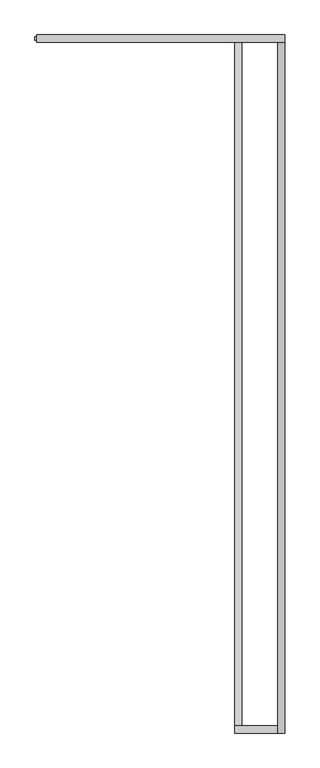
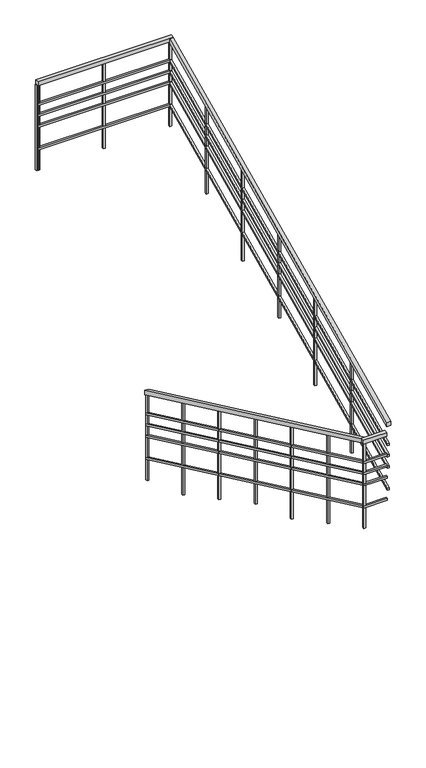
"""IFC4 building model written with IfcOpenShell, lengths in millimetres: railing geometry."""

from ifc_helpers import new_model, si_unit, frame, origin, place, context, project, spatial, polyline, outline, extrude, source, transform, mapped, element, save


def railing_ccc11bfa(model_context):
    return source(origin(), model_context, "Body", "SweptSolid", [
        extrude(outline(polyline([(4259.5597612, 1346.4361595), (4259.5597612, 1291.1764706), (-515.4402388, 3538.2352941), (-515.4402388, 3593.494983), (4259.5597612, 1346.4361595)])), frame((14225.0, 0.0, 0.0), z_axis=(1.0, 0.0, 0.0), x_axis=(0.0, 1.0, 0.0)), (0.0, 0.0, 1.0), 50.0),
        extrude(outline(polyline([(14225.0, -565.4402388), (14225.0, -515.4402388), (14525.0, -515.4402388), (14525.0, -565.4402388), (14225.0, -565.4402388)])), frame((0.0, 0.0, 3550.0), z_axis=(0.0, 0.0, 1.0), x_axis=(1.0, 0.0, 0.0)), (0.0, 0.0, 1.0), 50.0),
        extrude(outline(polyline([(-565.4402388, 3679.4117647), (-565.4402388, 3734.6714536), (4234.5597612, 5993.494983), (4234.5597612, 5938.2352941), (-565.4402388, 3679.4117647)])), frame((14525.0, 0.0, 0.0), z_axis=(1.0, 0.0, 0.0), x_axis=(0.0, 1.0, 0.0)), (0.0, 0.0, 1.0), 50.0),
        extrude(outline(polyline([(14575.0, 4284.5597612), (14575.0, 4234.5597612), (12850.0, 4234.5597612), (12850.0, 4284.5597612), (14575.0, 4284.5597612)])), frame((0.0, 0.0, 5950.0), z_axis=(0.0, 0.0, 1.0), x_axis=(1.0, 0.0, 0.0)), (0.0, 0.0, 1.0), 50.0),
        extrude(outline(polyline([(4259.5597612, 1041.1764706), (4259.5597612, 1013.5466261), (-527.9402388, 3266.4878026), (-527.9402388, 3294.1176471), (4259.5597612, 1041.1764706)])), frame((14237.5, 0.0, 0.0), z_axis=(1.0, 0.0, 0.0), x_axis=(0.0, 1.0, 0.0)), (0.0, 0.0, 1.0), 25.0),
        extrude(outline(polyline([(14237.5, -552.9402388), (14237.5, -527.9402388), (14537.5, -527.9402388), (14537.5, -552.9402388), (14237.5, -552.9402388)])), frame((0.0, 0.0, 3275.0), z_axis=(0.0, 0.0, 1.0), x_axis=(1.0, 0.0, 0.0)), (0.0, 0.0, 1.0), 25.0),
        extrude(outline(polyline([(-552.9402388, 3407.6642732), (-552.9402388, 3435.2941176), (4247.0597612, 5694.1176471), (4247.0597612, 5666.4878026), (-552.9402388, 3407.6642732)])), frame((14537.5, 0.0, 0.0), z_axis=(1.0, 0.0, 0.0), x_axis=(0.0, 1.0, 0.0)), (0.0, 0.0, 1.0), 25.0),
        extrude(outline(polyline([(14562.5, 4272.0597612), (14562.5, 4247.0597612), (12850.0, 4247.0597612), (12850.0, 4272.0597612), (14562.5, 4272.0597612)])), frame((0.0, 0.0, 5675.0), z_axis=(0.0, 0.0, 1.0), x_axis=(1.0, 0.0, 0.0)), (0.0, 0.0, 1.0), 25.0),
        extrude(outline(polyline([(4259.5597612, 891.1764706), (4259.5597612, 863.5466261), (-527.9402388, 3116.4878026), (-527.9402388, 3144.1176471), (4259.5597612, 891.1764706)])), frame((14237.5, 0.0, 0.0), z_axis=(1.0, 0.0, 0.0), x_axis=(0.0, 1.0, 0.0)), (0.0, 0.0, 1.0), 25.0),
        extrude(outline(polyline([(14237.5, -552.9402388), (14237.5, -527.9402388), (14537.5, -527.9402388), (14537.5, -552.9402388), (14237.5, -552.9402388)])), frame((0.0, 0.0, 3125.0), z_axis=(0.0, 0.0, 1.0), x_axis=(1.0, 0.0, 0.0)), (0.0, 0.0, 1.0), 25.0),
        extrude(outline(polyline([(-552.9402388, 3257.6642732), (-552.9402388, 3285.2941176), (4247.0597612, 5544.1176471), (4247.0597612, 5516.4878026), (-552.9402388, 3257.6642732)])), frame((14537.5, 0.0, 0.0), z_axis=(1.0, 0.0, 0.0), x_axis=(0.0, 1.0, 0.0)), (0.0, 0.0, 1.0), 25.0),
        extrude(outline(polyline([(14562.5, 4272.0597612), (14562.5, 4247.0597612), (12850.0, 4247.0597612), (12850.0, 4272.0597612), (14562.5, 4272.0597612)])), frame((0.0, 0.0, 5525.0), z_axis=(0.0, 0.0, 1.0), x_axis=(1.0, 0.0, 0.0)), (0.0, 0.0, 1.0), 25.0),
        extrude(outline(polyline([(4259.5597612, 741.1764706), (4259.5597612, 713.5466261), (-527.9402388, 2966.4878026), (-527.9402388, 2994.1176471), (4259.5597612, 741.1764706)])), frame((14237.5, 0.0, 0.0), z_axis=(1.0, 0.0, 0.0), x_axis=(0.0, 1.0, 0.0)), (0.0, 0.0, 1.0), 25.0),
        extrude(outline(polyline([(14237.5, -552.9402388), (14237.5, -527.9402388), (14537.5, -527.9402388), (14537.5, -552.9402388), (14237.5, -552.9402388)])), frame((0.0, 0.0, 2975.0), z_axis=(0.0, 0.0, 1.0), x_axis=(1.0, 0.0, 0.0)), (0.0, 0.0, 1.0), 25.0),
        extrude(outline(polyline([(-552.9402388, 3107.6642732), (-552.9402388, 3135.2941176), (4247.0597612, 5394.1176471), (4247.0597612, 5366.4878026), (-552.9402388, 3107.6642732)])), frame((14537.5, 0.0, 0.0), z_axis=(1.0, 0.0, 0.0), x_axis=(0.0, 1.0, 0.0)), (0.0, 0.0, 1.0), 25.0),
        extrude(outline(polyline([(14562.5, 4272.0597612), (14562.5, 4247.0597612), (12850.0, 4247.0597612), (12850.0, 4272.0597612), (14562.5, 4272.0597612)])), frame((0.0, 0.0, 5375.0), z_axis=(0.0, 0.0, 1.0), x_axis=(1.0, 0.0, 0.0)), (0.0, 0.0, 1.0), 25.0),
        extrude(outline(polyline([(4259.5597612, 441.1764706), (4259.5597612, 413.5466261), (-527.9402388, 2666.4878026), (-527.9402388, 2694.1176471), (4259.5597612, 441.1764706)])), frame((14237.5, 0.0, 0.0), z_axis=(1.0, 0.0, 0.0), x_axis=(0.0, 1.0, 0.0)), (0.0, 0.0, 1.0), 25.0),
        extrude(outline(polyline([(14237.5, -552.9402388), (14237.5, -527.9402388), (14537.5, -527.9402388), (14537.5, -552.9402388), (14237.5, -552.9402388)])), frame((0.0, 0.0, 2675.0), z_axis=(0.0, 0.0, 1.0), x_axis=(1.0, 0.0, 0.0)), (0.0, 0.0, 1.0), 25.0),
        extrude(outline(polyline([(-552.9402388, 2807.6642732), (-552.9402388, 2835.2941176), (4247.0597612, 5094.1176471), (4247.0597612, 5066.4878026), (-552.9402388, 2807.6642732)])), frame((14537.5, 0.0, 0.0), z_axis=(1.0, 0.0, 0.0), x_axis=(0.0, 1.0, 0.0)), (0.0, 0.0, 1.0), 25.0),
        extrude(outline(polyline([(14562.5, 4272.0597612), (14562.5, 4247.0597612), (12850.0, 4247.0597612), (12850.0, 4272.0597612), (14562.5, 4272.0597612)])), frame((0.0, 0.0, 5075.0), z_axis=(0.0, 0.0, 1.0), x_axis=(1.0, 0.0, 0.0)), (0.0, 0.0, 1.0), 25.0),
        extrude(outline(polyline([(12862.5, 4272.0597612), (12862.5, 4247.0597612), (12837.5, 4247.0597612), (12837.5, 4272.0597612), (12862.5, 4272.0597612)])), frame((0.0, 0.0, 4800.0), z_axis=(0.0, 0.0, 1.0), x_axis=(1.0, 0.0, 0.0)), (0.0, 0.0, 1.0), 1150.0),
        extrude(outline(polyline([(13712.5, 4272.0597612), (13712.5, 4247.0597612), (13687.5, 4247.0597612), (13687.5, 4272.0597612), (13712.5, 4272.0597612)])), frame((0.0, 0.0, 4800.0), z_axis=(0.0, 0.0, 1.0), x_axis=(1.0, 0.0, 0.0)), (0.0, 0.0, 1.0), 1150.0),
        extrude(outline(polyline([(4247.0597612, 4800.0), (4247.0597612, 5944.1176471), (4272.0597612, 5955.8823529), (4272.0597612, 4800.0), (4247.0597612, 4800.0)])), frame((14537.5, 0.0, 0.0), z_axis=(1.0, 0.0, 0.0), x_axis=(0.0, 1.0, 0.0)), (0.0, 0.0, 1.0), 25.0),
        extrude(outline(polyline([(3447.0597612, 4376.4705882), (3447.0597612, 5567.6470588), (3472.0597612, 5579.4117647), (3472.0597612, 4376.4705882), (3447.0597612, 4376.4705882)])), frame((14537.5, 0.0, 0.0), z_axis=(1.0, 0.0, 0.0), x_axis=(0.0, 1.0, 0.0)), (0.0, 0.0, 1.0), 25.0),
        extrude(outline(polyline([(2647.0597612, 3952.9411765), (2647.0597612, 5191.1764706), (2672.0597612, 5202.9411765), (2672.0597612, 3952.9411765), (2647.0597612, 3952.9411765)])), frame((14537.5, 0.0, 0.0), z_axis=(1.0, 0.0, 0.0), x_axis=(0.0, 1.0, 0.0)), (0.0, 0.0, 1.0), 25.0),
        extrude(outline(polyline([(1847.0597612, 3670.5882353), (1847.0597612, 4814.7058824), (1872.0597612, 4826.4705882), (1872.0597612, 3670.5882353), (1847.0597612, 3670.5882353)])), frame((14537.5, 0.0, 0.0), z_axis=(1.0, 0.0, 0.0), x_axis=(0.0, 1.0, 0.0)), (0.0, 0.0, 1.0), 25.0),
        extrude(outline(polyline([(1047.0597612, 3247.0588235), (1047.0597612, 4438.2352941), (1072.0597612, 4450.0), (1072.0597612, 3247.0588235), (1047.0597612, 3247.0588235)])), frame((14537.5, 0.0, 0.0), z_axis=(1.0, 0.0, 0.0), x_axis=(0.0, 1.0, 0.0)), (0.0, 0.0, 1.0), 25.0),
        extrude(outline(polyline([(247.0597612, 2823.5294118), (247.0597612, 4061.7647059), (272.0597612, 4073.5294118), (272.0597612, 2823.5294118), (247.0597612, 2823.5294118)])), frame((14537.5, 0.0, 0.0), z_axis=(1.0, 0.0, 0.0), x_axis=(0.0, 1.0, 0.0)), (0.0, 0.0, 1.0), 25.0),
        extrude(outline(polyline([(-527.9402388, 3544.1176471), (-527.9402388, 2400.0), (-552.9402388, 2400.0), (-552.9402388, 3555.8823529), (-527.9402388, 3544.1176471)])), frame((14237.5, 0.0, 0.0), z_axis=(1.0, 0.0, 0.0), x_axis=(0.0, 1.0, 0.0)), (0.0, 0.0, 1.0), 25.0),
        extrude(outline(polyline([(272.0597612, 3167.6470588), (272.0597612, 1976.4705882), (247.0597612, 1976.4705882), (247.0597612, 3179.4117647), (272.0597612, 3167.6470588)])), frame((14237.5, 0.0, 0.0), z_axis=(1.0, 0.0, 0.0), x_axis=(0.0, 1.0, 0.0)), (0.0, 0.0, 1.0), 25.0),
        extrude(outline(polyline([(1072.0597612, 2791.1764706), (1072.0597612, 1552.9411765), (1047.0597612, 1552.9411765), (1047.0597612, 2802.9411765), (1072.0597612, 2791.1764706)])), frame((14237.5, 0.0, 0.0), z_axis=(1.0, 0.0, 0.0), x_axis=(0.0, 1.0, 0.0)), (0.0, 0.0, 1.0), 25.0),
        extrude(outline(polyline([(1872.0597612, 2414.7058824), (1872.0597612, 1270.5882353), (1847.0597612, 1270.5882353), (1847.0597612, 2426.4705882), (1872.0597612, 2414.7058824)])), frame((14237.5, 0.0, 0.0), z_axis=(1.0, 0.0, 0.0), x_axis=(0.0, 1.0, 0.0)), (0.0, 0.0, 1.0), 25.0),
        extrude(outline(polyline([(2672.0597612, 2038.2352941), (2672.0597612, 847.0588235), (2647.0597612, 847.0588235), (2647.0597612, 2050.0), (2672.0597612, 2038.2352941)])), frame((14237.5, 0.0, 0.0), z_axis=(1.0, 0.0, 0.0), x_axis=(0.0, 1.0, 0.0)), (0.0, 0.0, 1.0), 25.0),
        extrude(outline(polyline([(3472.0597612, 1661.7647059), (3472.0597612, 423.5294118), (3447.0597612, 423.5294118), (3447.0597612, 1673.5294118), (3472.0597612, 1661.7647059)])), frame((14237.5, 0.0, 0.0), z_axis=(1.0, 0.0, 0.0), x_axis=(0.0, 1.0, 0.0)), (0.0, 0.0, 1.0), 25.0),
        extrude(outline(polyline([(12875.0, 4272.0597612), (12875.0, 4247.0597612), (12850.0, 4247.0597612), (12850.0, 4272.0597612), (12875.0, 4272.0597612)])), frame((0.0, 0.0, 4800.0), z_axis=(0.0, 0.0, 1.0), x_axis=(1.0, 0.0, 0.0)), (0.0, 0.0, 1.0), 1150.0),
        extrude(outline(polyline([(4259.5597612, 1291.1764706), (4259.5597612, 141.1764706), (4234.5597612, 141.1764706), (4234.5597612, 1302.9411765), (4259.5597612, 1291.1764706)])), frame((14237.5, 0.0, 0.0), z_axis=(1.0, 0.0, 0.0), x_axis=(0.0, 1.0, 0.0)), (0.0, 0.0, 1.0), 25.0),
    ])


if __name__ == "__main__":
    model = new_model("IFC4")
    model_context = context("Model", 3, world=origin())
    ifc_project = project(units=[si_unit("LENGTHUNIT", "METRE", prefix="MILLI")], contexts=[model_context])
    site = spatial("IfcSite", under=ifc_project)
    building = spatial("IfcBuilding", under=site)
    placement = place(None, origin())
    railing_shape = railing_ccc11bfa(model_context)
    element("IfcRailing", 1, at=placement, inside=building, context=model_context, shape_type="MappedRepresentation", body=[
        mapped(railing_shape, transform((0.0, 0.0, 0.0), x_axis=(1.0, 0.0, 0.0), y_axis=(0.0, 1.0, 0.0), z_axis=(0.0, 0.0, 1.0))),
    ])
    save(model, "model.ifc")
